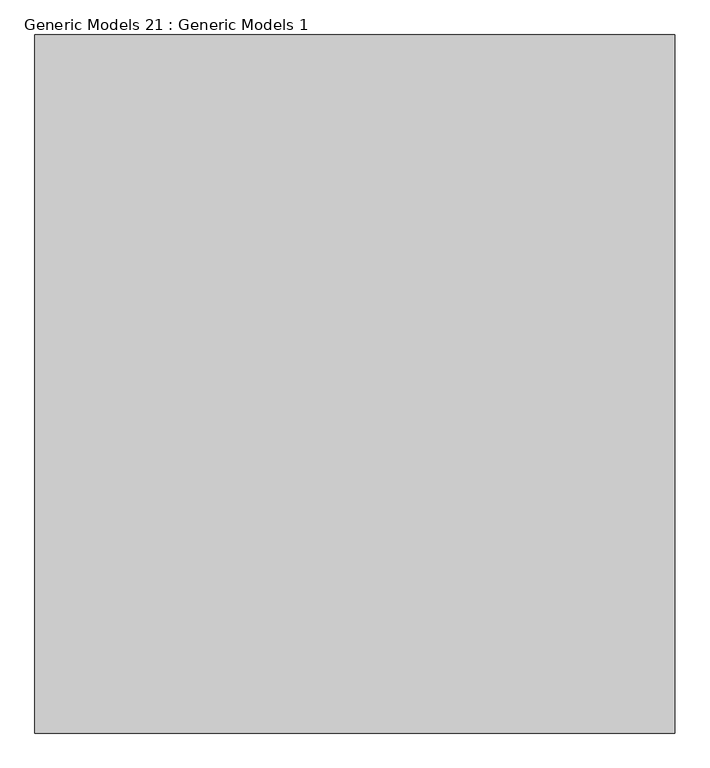
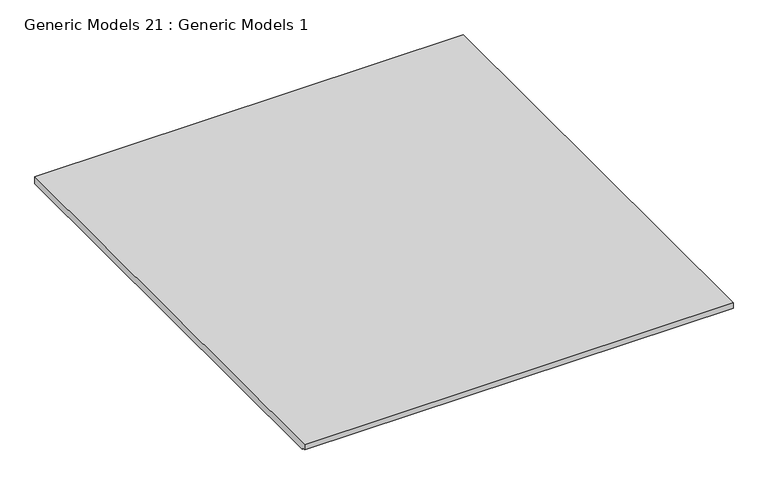
"""IFC4 building model written with IfcOpenShell, lengths in millimetres: proxy geometry, Generic Models 21 : Generic Models 1."""

from ifc_helpers import new_model, si_unit, frame, origin, place, context, project, spatial, polyline, outline, extrude, source, transform, mapped, element, save


def generic_models_21_generic_models_1_464872a0(model_context):
    return source(origin(), model_context, "Body", "SweptSolid", [
        extrude(outline(polyline([(39621.7705945, 2631.6803942), (40840.9705945, 2631.6803942), (40840.9705945, 2612.6303942), (39632.7637259, 2612.6303942), (39632.7637259, 2617.3928942), (39621.7705945, 2617.3928942), (39621.7705945, 2631.6803942)])), frame((51480.3077305, 0.0, 0.0), z_axis=(1.0, 0.0, 0.0), x_axis=(0.0, 1.0, 0.0)), (0.0, 0.0, 1.0), 1117.6),
    ])


if __name__ == "__main__":
    model = new_model("IFC4")
    model_context = context("Model", 3, world=origin())
    ifc_project = project(units=[si_unit("LENGTHUNIT", "METRE", prefix="MILLI")], contexts=[model_context])
    site = spatial("IfcSite", under=ifc_project)
    building = spatial("IfcBuilding", under=site)
    placement = place(None, origin())
    generic_models_21_generic_models_1_shape = generic_models_21_generic_models_1_464872a0(model_context)
    element("IfcBuildingElementProxy", 1, Name="Generic Models 21 : Generic Models 1", ObjectType="Generic Models 21 : Generic Models 1", at=placement, inside=building, context=model_context, shape_type="MappedRepresentation", body=[
        mapped(generic_models_21_generic_models_1_shape, transform((0.0, 0.0, 0.0), x_axis=(1.0, 0.0, 0.0), y_axis=(0.0, 1.0, 0.0), z_axis=(0.0, 0.0, 1.0))),
    ])
    save(model, "model.ifc")

# Revit data of these elements
# Element 1 (IfcBuildingElementProxy, "Generic Models 21 : Generic Models 1")
#   Materials on its faces: "EXISTING ACOUSTICAL TILE"
# Materials
#   "EXISTING ACOUSTICAL TILE": class "Generic", colour RGB 120 120 120, transparency 0, Cost = 0
